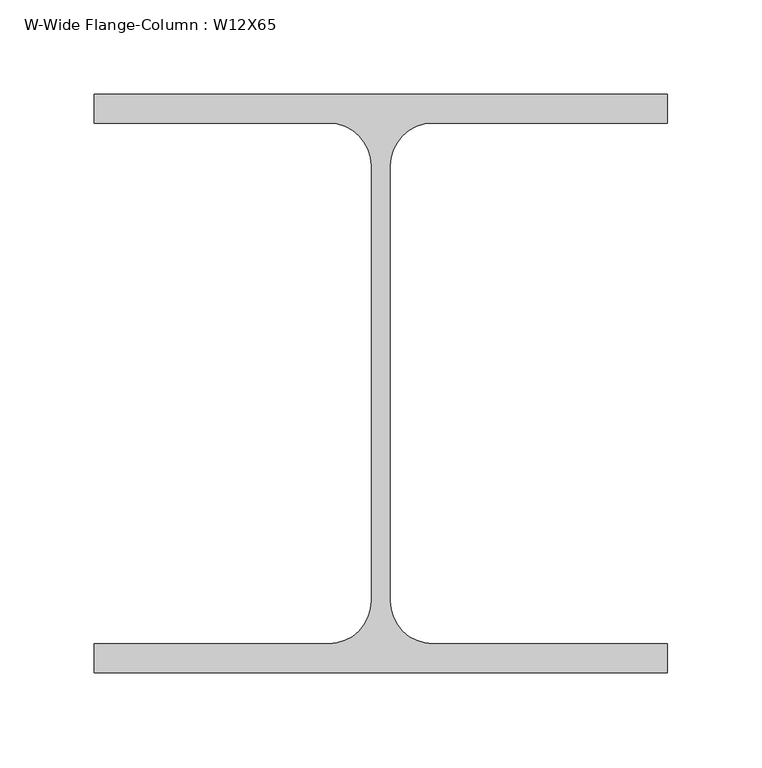
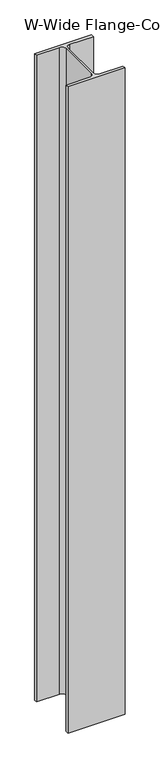
"""IFC4 building model written with IfcOpenShell, lengths in millimetres: column geometry, W-Wide Flange-Column : W12X65."""

from ifc_helpers import new_model, si_unit, point, frame, frame_2d, origin, place, context, project, spatial, polyline, circle_curve, trimmed, segment, composite_curve, outline, extrude, source, transform, mapped, element, save


def w_wide_flange_column_w12x65_2ed8671b(model_context):
    return source(origin(), model_context, "Body", "SweptSolid", [
        extrude(outline(composite_curve([segment(polyline([(152.4, 153.67), (152.4, 138.303), (27.686, 138.303)]), True, "CONTINUOUS"), segment(trimmed(circle_curve(frame_2d((27.686, 115.57)), 22.733), [point((27.686, 138.303))], [point((4.953, 115.57))], True, "CARTESIAN"), True, "CONTINUOUS"), segment(polyline([(4.953, 115.57), (4.953, -115.57)]), True, "CONTINUOUS"), segment(trimmed(circle_curve(frame_2d((27.686, -115.57)), 22.733), [point((4.953, -115.57))], [point((27.686, -138.303))], True, "CARTESIAN"), True, "CONTINUOUS"), segment(polyline([(27.686, -138.303), (152.4, -138.303), (152.4, -153.67), (-152.4, -153.67), (-152.4, -138.303), (-27.686, -138.303)]), True, "CONTINUOUS"), segment(trimmed(circle_curve(frame_2d((-27.686, -115.57)), 22.733), [point((-27.686, -138.303))], [point((-4.953, -115.57))], True, "CARTESIAN"), True, "CONTINUOUS"), segment(polyline([(-4.953, -115.57), (-4.953, 115.57)]), True, "CONTINUOUS"), segment(trimmed(circle_curve(frame_2d((-27.686, 115.57)), 22.733), [point((-4.953, 115.57))], [point((-27.686, 138.303))], True, "CARTESIAN"), True, "CONTINUOUS"), segment(polyline([(-27.686, 138.303), (-152.4, 138.303), (-152.4, 153.67), (152.4, 153.67)]), True, "CONTINUOUS")], self_intersect=False)), frame((0.0, 0.0, 8756.65), z_axis=(0.0, 0.0, 1.0), x_axis=(1.0, 0.0, 0.0)), (0.0, 0.0, 1.0), 3651.25),
    ])


if __name__ == "__main__":
    model = new_model("IFC4")
    model_context = context("Model", 3, world=origin())
    ifc_project = project(units=[si_unit("LENGTHUNIT", "METRE", prefix="MILLI")], contexts=[model_context])
    site = spatial("IfcSite", under=ifc_project)
    building = spatial("IfcBuilding", under=site)
    placement = place(None, origin())
    w_wide_flange_column_w12x65_shape = w_wide_flange_column_w12x65_2ed8671b(model_context)
    element("IfcColumn", 1, ObjectType="W-Wide Flange-Column : W12X65", at=placement, inside=building, context=model_context, shape_type="MappedRepresentation", body=[
        mapped(w_wide_flange_column_w12x65_shape, transform((0.0, 0.0, 0.0), x_axis=(1.0, 0.0, 0.0), y_axis=(0.0, 1.0, 0.0), z_axis=(0.0, 0.0, 1.0))),
    ])
    save(model, "model.ifc")

# Revit data of these elements
# Type "W-Wide Flange-Column : W12X65"
#   Assembly Code = "B10"
#   W = 65
#   bf = 1' - 0"
#   d = 1' - 0.1"
#   k = 0' - 1 1/2"
#   kr = 0' - 0.895"
#   tf = 0' - 0.605"
#   tw = 0' - 0.39"
#   A = 0.132639 SF
#   Structural Material [instance default] = Steel ASTM A992
# Element 1 (IfcColumn, "W-Wide Flange-Column : W12X65")
#   Materials on its faces: "Steel ASTM A992"
# Materials
#   "Steel ASTM A992": class "Metal", colour RGB 199 199 199, transparency 0, Description = "Structural steel 50ksi", Cost = 0
